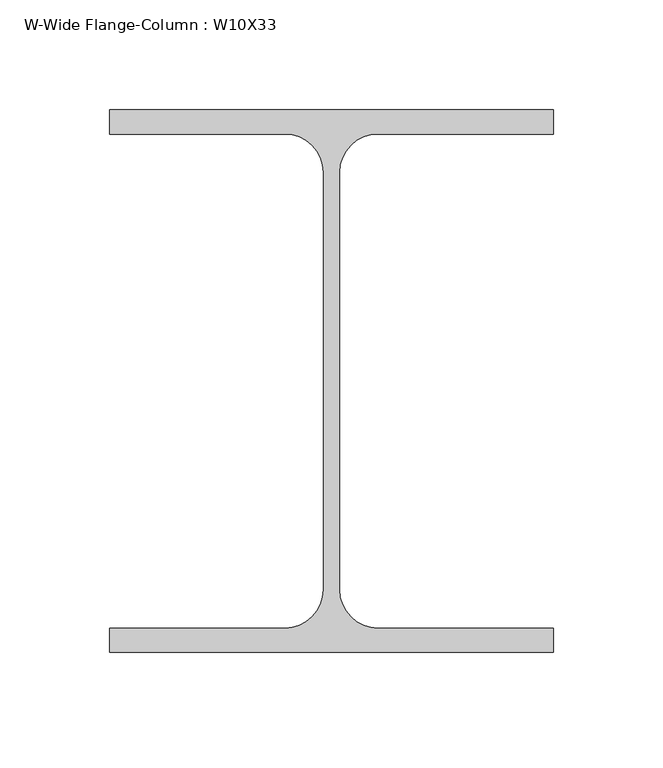
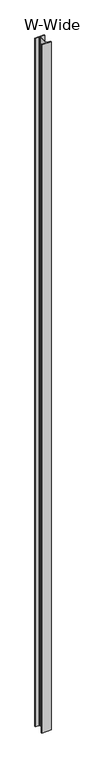
"""IFC4 building model written with IfcOpenShell, lengths in millimetres: column geometry, W-Wide Flange-Column : W10X33."""

from ifc_helpers import new_model, si_unit, point, frame, frame_2d, origin, place, context, project, spatial, polyline, circle_curve, trimmed, segment, composite_curve, outline, extrude, source, transform, mapped, element, save


def w_wide_flange_column_w10x33_b445f528(model_context):
    return source(origin(), model_context, "Body", "SweptSolid", [
        extrude(outline(composite_curve([segment(polyline([(101.092, 123.571), (101.092, 112.522), (21.209, 112.522)]), True, "CONTINUOUS"), segment(trimmed(circle_curve(frame_2d((21.209, 94.996)), 17.526), [point((21.209, 112.522))], [point((3.683, 94.996))], True, "CARTESIAN"), True, "CONTINUOUS"), segment(polyline([(3.683, 94.996), (3.683, -94.996)]), True, "CONTINUOUS"), segment(trimmed(circle_curve(frame_2d((21.209, -94.996)), 17.526), [point((3.683, -94.996))], [point((21.209, -112.522))], True, "CARTESIAN"), True, "CONTINUOUS"), segment(polyline([(21.209, -112.522), (101.092, -112.522), (101.092, -123.571), (-101.092, -123.571), (-101.092, -112.522), (-21.209, -112.522)]), True, "CONTINUOUS"), segment(trimmed(circle_curve(frame_2d((-21.209, -94.996)), 17.526), [point((-21.209, -112.522))], [point((-3.683, -94.996))], True, "CARTESIAN"), True, "CONTINUOUS"), segment(polyline([(-3.683, -94.996), (-3.683, 94.996)]), True, "CONTINUOUS"), segment(trimmed(circle_curve(frame_2d((-21.209, 94.996)), 17.526), [point((-3.683, 94.996))], [point((-21.209, 112.522))], True, "CARTESIAN"), True, "CONTINUOUS"), segment(polyline([(-21.209, 112.522), (-101.092, 112.522), (-101.092, 123.571), (101.092, 123.571)]), True, "CONTINUOUS")], self_intersect=False)), frame((0.0, 0.0, 8756.65), z_axis=(0.0, 0.0, 1.0), x_axis=(1.0, 0.0, 0.0)), (0.0, 0.0, 1.0), 15584.1898438),
    ])


if __name__ == "__main__":
    model = new_model("IFC4")
    model_context = context("Model", 3, world=origin())
    ifc_project = project(units=[si_unit("LENGTHUNIT", "METRE", prefix="MILLI")], contexts=[model_context])
    site = spatial("IfcSite", under=ifc_project)
    building = spatial("IfcBuilding", under=site)
    placement = place(None, origin())
    w_wide_flange_column_w10x33_shape = w_wide_flange_column_w10x33_b445f528(model_context)
    element("IfcColumn", 1, ObjectType="W-Wide Flange-Column : W10X33", at=placement, inside=building, context=model_context, shape_type="MappedRepresentation", body=[
        mapped(w_wide_flange_column_w10x33_shape, transform((0.0, 0.0, 0.0), x_axis=(1.0, 0.0, 0.0), y_axis=(0.0, 1.0, 0.0), z_axis=(0.0, 0.0, 1.0))),
    ])
    save(model, "model.ifc")

# Revit data of these elements
# Type "W-Wide Flange-Column : W10X33"
#   Assembly Code = "B10"
#   W = 33
#   bf = 0' - 7.96"
#   d = 0' - 9.73"
#   k = 0' - 1 1/8"
#   kr = 0' - 0.69"
#   tf = 0' - 0.435"
#   tw = 0' - 0.29"
#   A = 0.0674306 SF
#   Structural Material [instance default] = Steel ASTM A992
# Element 1 (IfcColumn, "W-Wide Flange-Column : W10X33")
#   Materials on its faces: "Steel ASTM A992"
# Materials
#   "Steel ASTM A992": class "Metal", colour RGB 199 199 199, transparency 0, Description = "Structural steel 50ksi", Cost = 0
